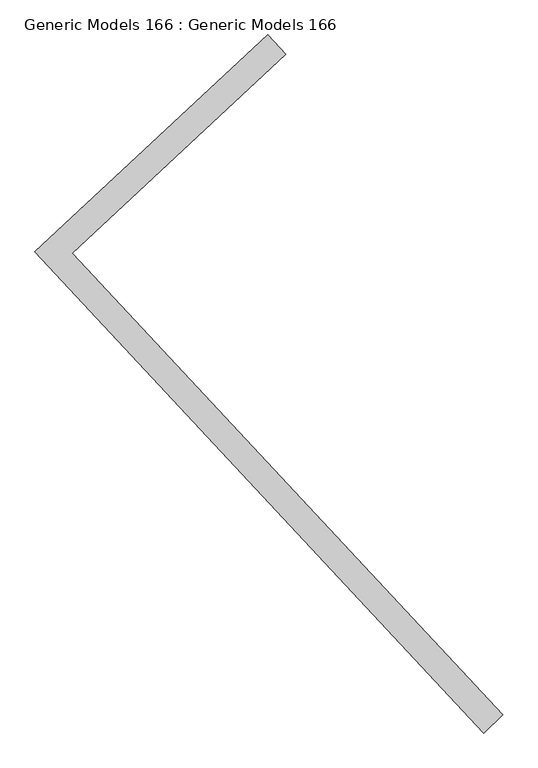
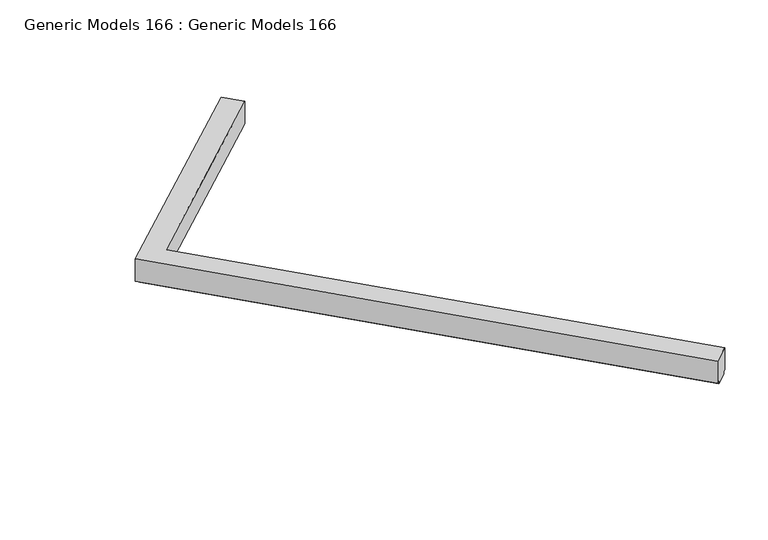
"""IFC4 building model written with IfcOpenShell, lengths in millimetres: proxy geometry, Generic Models 166 : Generic Models 166."""

from ifc_helpers import new_model, si_unit, origin, place, context, project, spatial, faceted_brep, source, transform, mapped, element, save


def generic_models_166_generic_models_166_05eff111(model_context):
    return source(origin(), model_context, "Body", "Brep", [
        faceted_brep([(5594.1695075, -15059.4810027, 2239.565625), (5680.7832992, -15152.3629228, 2239.565625), (5680.7832992, -15152.3629228, 2099.865625), (5667.7912305, -15138.4306348, 2099.865625), (5667.7912305, -15138.4306348, 2082.8), (5607.1615763, -15073.4132907, 2082.8), (5607.1615763, -15073.4132907, 2099.865625), (5594.1695075, -15059.4810027, 2099.865625), (6627.6085011, -18402.318122, 2239.565625), (6627.6085011, -18402.318122, 2099.865625), (6641.5407891, -18389.3260533, 2099.865625), (6641.5407891, -18389.3260533, 2082.8), (6706.5581332, -18328.6963991, 2082.8), (6706.5581332, -18328.6963991, 2099.865625), (6720.4904212, -18315.7043303, 2099.865625), (6720.4904212, -18315.7043303, 2239.565625), (4479.5864662, -16098.8465034, 2239.565625), (4659.0821781, -16105.1146318, 2239.565625), (4659.0821781, -16105.1146318, 2099.865625), (4632.1578213, -16104.1744125, 2099.865625), (4632.1578213, -16104.1744125, 2082.8), (4506.510823, -16099.7867227, 2082.8), (4506.510823, -16099.7867227, 2099.865625), (4479.5864662, -16098.8465034, 2099.865625)], [[[0, 1, 2, 3, 4, 5, 6, 7]], [[8, 9, 10, 11, 12, 13, 14, 15]], [[1, 0, 16, 8, 15, 17]], [[2, 1, 17, 18]], [[3, 2, 18, 14, 13, 19]], [[4, 3, 19, 20]], [[5, 4, 20, 12, 11, 21]], [[6, 5, 21, 22]], [[7, 6, 22, 10, 9, 23]], [[0, 7, 23, 16]], [[18, 17, 15, 14]], [[20, 19, 13, 12]], [[22, 21, 11, 10]], [[16, 23, 9, 8]]]),
    ])


if __name__ == "__main__":
    model = new_model("IFC4")
    model_context = context("Model", 3, world=origin())
    ifc_project = project(units=[si_unit("LENGTHUNIT", "METRE", prefix="MILLI")], contexts=[model_context])
    site = spatial("IfcSite", under=ifc_project)
    building = spatial("IfcBuilding", under=site)
    placement = place(None, origin())
    generic_models_166_generic_models_166_shape = generic_models_166_generic_models_166_05eff111(model_context)
    element("IfcBuildingElementProxy", 1, Name="Generic Models 166 : Generic Models 166", ObjectType="Generic Models 166 : Generic Models 166", at=placement, inside=building, context=model_context, shape_type="MappedRepresentation", body=[
        mapped(generic_models_166_generic_models_166_shape, transform((0.0, 0.0, 0.0), x_axis=(1.0, 0.0, 0.0), y_axis=(0.0, 1.0, 0.0), z_axis=(0.0, 0.0, 1.0))),
    ])
    save(model, "model.ifc")

# Revit data of these elements
# Element 1 (IfcBuildingElementProxy, "Generic Models 166 : Generic Models 166")
#   Materials on its faces: "1 x 6 WOOD TRIM"
# Materials
#   "1 x 6 WOOD TRIM": class "Wood", colour RGB 48 37 22, transparency 0, Description = "Pinus Echinata", Cost = 0
